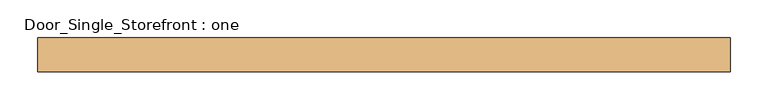
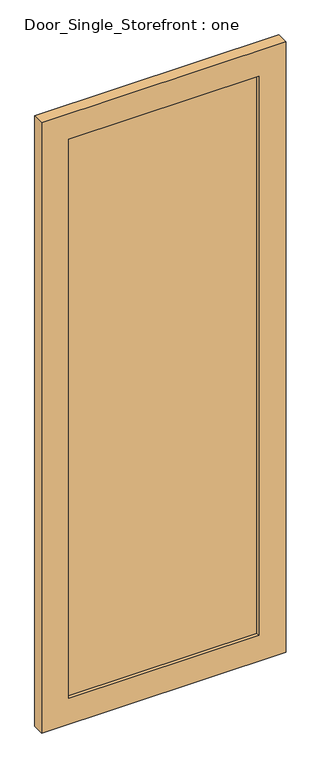
"""IFC4 building model written with IfcOpenShell, lengths in millimetres: door geometry, Door_Single_Storefront : one."""

from ifc_helpers import new_model, si_unit, frame, origin, place, context, project, spatial, polyline, outline, extrude, source, transform, mapped, element, save


def door_single_storefront_one_01d8a243(model_context):
    return source(origin(), model_context, "Body", "SweptSolid", [
        extrude(outline(polyline([(355.6, -19.05), (355.6, -38.1), (-355.6, -38.1), (-355.6, -19.05), (355.6, -19.05)])), frame((0.0, 0.0, 101.6), z_axis=(0.0, 0.0, 1.0), x_axis=(1.0, 0.0, 0.0)), (0.0, 0.0, 1.0), 2209.8),
        extrude(outline(polyline([(2413.0, -457.2), (0.0, -457.2), (0.0, 457.2), (2413.0, 457.2), (2413.0, -457.2)]), holes=[polyline([(101.6, 355.6), (101.6, -355.6), (2311.4, -355.6), (2311.4, 355.6), (101.6, 355.6)])]), frame((0.0, -50.8, 0.0), z_axis=(0.0, 1.0, 0.0), x_axis=(0.0, 0.0, 1.0)), (0.0, 0.0, 1.0), 44.45),
    ])


if __name__ == "__main__":
    model = new_model("IFC4")
    model_context = context("Model", 3, world=origin())
    ifc_project = project(units=[si_unit("LENGTHUNIT", "METRE", prefix="MILLI")], contexts=[model_context])
    site = spatial("IfcSite", under=ifc_project)
    building = spatial("IfcBuilding", under=site)
    placement = place(None, origin())
    door_single_storefront_one_shape = door_single_storefront_one_01d8a243(model_context)
    element("IfcDoor", 1, ObjectType="Door_Single_Storefront : one", at=placement, inside=building, context=model_context, shape_type="MappedRepresentation", body=[
        mapped(door_single_storefront_one_shape, transform((0.0, 0.0, 0.0), x_axis=(1.0, 0.0, 0.0), y_axis=(0.0, 1.0, 0.0), z_axis=(0.0, 0.0, 1.0))),
    ])
    save(model, "model.ifc")

# Revit data of these elements
# Type "Door_Single_Storefront : one"
#   Type Mark = "27"
#   Analytic Construction = "<None>"
#   Stile_Width = 0' - 4"
#   Door_Thickness = 0' - 1 3/4"
#   Door_Offset = 0' - 2"
#   Glass_Material = Glass
#   Frame_Material = Aluminum
#   Function = (empty or 0)
# Element 1 (IfcDoor, "Door_Single_Storefront : one")
#   Materials on its faces: "Aluminum", "Glass"
# Materials
#   "Glass": class "Glass", colour RGB 0 128 192, transparency 0.75, Description = "Soda Lime Glass", Cost = 0
#   "Aluminum": class "Metal", colour RGB 247 247 247, transparency 0, Description = "Aluminum 6061", Cost = 0
